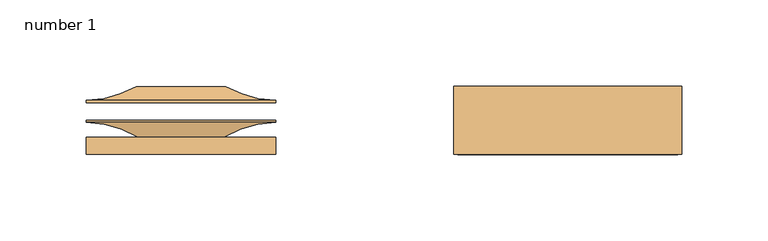
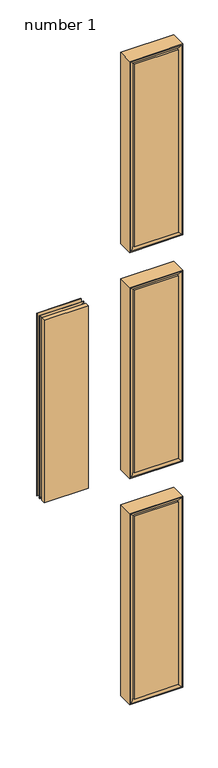
"""IFC4 building model written with IfcOpenShell, lengths in millimetres: door geometry, Door-Interior-Karona-K5660-6_Panel : number 1."""

from ifc_helpers import new_model, si_unit, frame, origin, place, context, project, spatial, polyline, ellipse_curve, source, transform, mapped, element, save
from ifc_brep_helpers import plane_surface, cylinder_surface, revolved_surface, advanced_brep


def number_1_6f4e57e8(model_context):
    return source(origin(), model_context, "Body", "AdvancedBrep", [
        advanced_brep(
        [(166.6748, -54.4576, 1893.8748), (57.1627, -54.4576, 1893.8748), (57.1627, -54.4576, 1414.4752), (166.6748, -54.4576, 1414.4752), (166.6748, -34.7218, 1893.8748), (57.1627, -34.7218, 1893.8748), (57.1627, -36.0454899, 1893.8748), (166.6748, -36.0454899, 1893.8748), (166.6748, -44.5515929, 1893.8748), (57.1627, -44.5515929, 1893.8748), (57.1627, -34.7218, 1414.4752), (166.6748, -34.7218, 1414.4752), (166.6748, -36.0454899, 1414.4752), (57.1627, -36.0454899, 1414.4752), (57.1627, -44.5515929, 1414.4752), (166.6748, -44.5515929, 1414.4752), (87.1686653, -44.5515929, 1863.8688347), (136.6688347, -44.5515929, 1863.8688347), (87.1686653, -44.5515929, 1444.4811653), (136.6688347, -44.5515929, 1444.4811653)],
        [
            (0, 1),
            (1, 2),
            (2, 3),
            (3, 0),
            (4, 5),
            (5, 6),
            (6, 7),
            (7, 4),
            (0, 8),
            (8, 9),
            (9, 1),
            (10, 11),
            (11, 12),
            (12, 13),
            (13, 10),
            (2, 14),
            (14, 15),
            (15, 3),
            (15, 8),
            (11, 4),
            (7, 12),
            (9, 14),
            (5, 10),
            (13, 6),
            (16, 17),
            (17, 7, ellipse_curve(frame((168.6131685, -100.0605261, 1895.8131685), z_axis=(0.7071067811865475, 0.0, -0.7071067811865475), x_axis=(0.7071067811865476, 0.0, 0.7071067811865474)), 90.5724254, 64.0443762)),
            (6, 16, ellipse_curve(frame((55.2243315, -100.0605261, 1895.8131685), z_axis=(-0.7071067811865475, 0.0, -0.7071067811865475), x_axis=(0.7071067811865476, 0.0, -0.7071067811865474)), 90.5724254, 64.0443762)),
            (18, 16),
            (13, 18, ellipse_curve(frame((55.2243315, -100.0605261, 1412.5368315), z_axis=(0.7071067811865475, 0.0, -0.7071067811865475), x_axis=(0.7071067811865474, 0.0, 0.7071067811865476)), 90.5724254, 64.0443762)),
            (19, 18),
            (12, 19, ellipse_curve(frame((168.6131685, -100.0605261, 1412.5368315), z_axis=(0.7071067811865475, 0.0, 0.7071067811865475), x_axis=(-0.7071067811865476, 0.0, 0.7071067811865474)), 90.5724254, 64.0443762)),
            (17, 19),
        ],
        [
            plane_surface(frame((57.1627, -54.4576, 1893.8748), z_axis=(0.0, -1.0, 0.0), x_axis=(0.0, 0.0, -1.0))),
            plane_surface(frame((57.1627, -34.7218, 1893.8748), z_axis=(0.0, 0.0, 1.0), x_axis=(-1.0, 0.0, 0.0))),
            plane_surface(frame((57.1627, -34.7218, 1414.4752), z_axis=(0.0, 0.0, -1.0), x_axis=(1.0, 0.0, 0.0))),
            plane_surface(frame((166.6748, -54.4576, 1893.8748), z_axis=(1.0, 0.0, 0.0), x_axis=(0.0, 0.0, -1.0))),
            plane_surface(frame((57.1627, -34.7218, 1893.8748), z_axis=(-1.0, 0.0, 0.0), x_axis=(0.0, 0.0, -1.0))),
            plane_surface(frame((166.6748, -34.7218, 1893.8748), z_axis=(0.0, 1.0, 0.0), x_axis=(0.0, 0.0, -1.0))),
            revolved_surface(polyline([(232.6575446888527, -100.0605261, 1831.7687923), (-8.820044688852704, -100.0605261, 1831.7687923)]), (177.8, -100.0605261, 1895.8131685), (1.0, 0.0, 0.0)),
            revolved_surface(polyline([(119.2687077, -100.0605261, 1959.8575446888528), (119.2687077, -100.0605261, 1348.4924553111473)]), (55.2243315, -100.0605261, 1905.0), (0.0, 0.0, 1.0)),
            revolved_surface(polyline([(-8.820044688852683, -100.0605261, 1476.5812077), (232.6575446888527, -100.0605261, 1476.5812077)]), (46.0375, -100.0605261, 1412.5368315), (-1.0, 0.0, 0.0)),
            revolved_surface(polyline([(104.5687923, -100.0605261, 1348.4924553111473), (104.5687923, -100.0605261, 1959.8575446888526)]), (168.6131685, -100.0605261, 1403.35), (0.0, 0.0, -1.0)),
            plane_surface(frame((177.8, -44.5515929, 1403.35), z_axis=(0.0, 1.0, 0.0), x_axis=(0.0, 0.0, 1.0))),
        ],
        [
            (0, [[1, 2, 3, 4]]),
            (1, [[5, 6, 7, 8]]),
            (1, [[-1, 9, 10, 11]]),
            (2, [[12, 13, 14, 15]]),
            (2, [[-3, 16, 17, 18]]),
            (3, [[-4, -18, 19, -9]]),
            (3, [[20, -8, 21, -13]]),
            (4, [[-2, -11, 22, -16]]),
            (4, [[23, -15, 24, -6]]),
            (5, [[-5, -20, -12, -23]]),
            (6, [[25, 26, -7, 27]]),
            (7, [[28, -27, -24, 29]]),
            (8, [[30, -29, -14, 31]]),
            (9, [[32, -31, -21, -26]]),
            (10, [[-10, -19, -17, -22], [-25, -28, -30, -32]]),
        ],
    ),
        advanced_brep(
        [(166.6748, -24.6126, 1893.8748), (57.1627, -24.6126, 1893.8748), (57.1627, -24.6126, 1414.4752), (166.6748, -24.6126, 1414.4752), (137.8448579, -15.4432, 1443.3051421), (85.9926421, -15.4432, 1443.3051421), (85.9926421, -15.4432, 1865.0448579), (137.8448579, -15.4432, 1865.0448579), (166.6748, -23.2889101, 1893.8748), (57.1627, -23.2889101, 1893.8748), (57.1627, -23.2889101, 1414.4752), (166.6748, -23.2889101, 1414.4752)],
        [
            (0, 1),
            (1, 2),
            (2, 3),
            (3, 0),
            (4, 5),
            (5, 6),
            (6, 7),
            (7, 4),
            (0, 8),
            (8, 9),
            (9, 1),
            (2, 10),
            (10, 11),
            (11, 3),
            (4, 11, ellipse_curve(frame((168.6131685, 40.7261261, 1412.5368315), z_axis=(0.7071067811865475, 0.0, 0.7071067811865475), x_axis=(-0.7071067811865476, 0.0, 0.7071067811865474)), 90.5724254, 64.0443762)),
            (10, 5, ellipse_curve(frame((55.2243315, 40.7261261, 1412.5368315), z_axis=(-0.7071067811865475, 0.0, 0.7071067811865475), x_axis=(-0.7071067811865476, 0.0, -0.7071067811865474)), 90.5724254, 64.0443762)),
            (7, 8, ellipse_curve(frame((168.6131685, 40.7261261, 1895.8131685), z_axis=(-0.7071067811865475, 0.0, 0.7071067811865475), x_axis=(-0.7071067811865474, 0.0, -0.7071067811865476)), 90.5724254, 64.0443762)),
            (8, 11),
            (6, 9, ellipse_curve(frame((55.2243315, 40.7261261, 1895.8131685), z_axis=(-0.7071067811865475, 0.0, -0.7071067811865475), x_axis=(0.7071067811865476, 0.0, -0.7071067811865474)), 90.5724254, 64.0443762)),
            (10, 9),
        ],
        [
            plane_surface(frame((57.1627, -24.6126, 1893.8748), z_axis=(0.0, -1.0, 0.0), x_axis=(0.0, 0.0, -1.0))),
            plane_surface(frame((166.6748, -15.4432, 1893.8748), z_axis=(0.0, 1.0, 0.0), x_axis=(0.0, 0.0, -1.0))),
            plane_surface(frame((57.1627, -34.7218, 1893.8748), z_axis=(0.0, 0.0, 1.0), x_axis=(-1.0, 0.0, 0.0))),
            plane_surface(frame((57.1627, -34.7218, 1414.4752), z_axis=(0.0, 0.0, -1.0), x_axis=(1.0, 0.0, 0.0))),
            revolved_surface(polyline([(-8.820044688852711, 40.7261261, 1476.5812077), (232.6575446888527, 40.7261261, 1476.5812077)]), (46.0375, 40.7261261, 1412.5368315), (-1.0, 0.0, 0.0)),
            revolved_surface(polyline([(104.5687923, 40.7261261, 1348.4924553111473), (104.5687923, 40.7261261, 1959.8575446888528)]), (168.6131685, 40.7261261, 1403.35), (0.0, 0.0, -1.0)),
            revolved_surface(polyline([(232.65754468885268, 40.7261261, 1831.7687923), (-8.820044688852704, 40.7261261, 1831.7687923)]), (177.8, 40.7261261, 1895.8131685), (1.0, 0.0, 0.0)),
            revolved_surface(polyline([(119.2687077, 40.7261261, 1959.8575446888528), (119.2687077, 40.7261261, 1348.4924553111473)]), (55.2243315, 40.7261261, 1905.0), (0.0, 0.0, 1.0)),
            plane_surface(frame((166.6748, -24.6126, 1893.8748), z_axis=(1.0, 0.0, 0.0), x_axis=(0.0, 0.0, -1.0))),
            plane_surface(frame((57.1627, -15.4432, 1893.8748), z_axis=(-1.0, 0.0, 0.0), x_axis=(0.0, 0.0, -1.0))),
        ],
        [
            (0, [[1, 2, 3, 4]]),
            (1, [[5, 6, 7, 8]]),
            (2, [[-1, 9, 10, 11]]),
            (3, [[-3, 12, 13, 14]]),
            (4, [[15, -13, 16, -5]]),
            (5, [[-15, -8, 17, 18]]),
            (6, [[-17, -7, 19, -10]]),
            (7, [[-19, -6, -16, 20]]),
            (8, [[-4, -14, -18, -9]]),
            (9, [[-2, -11, -20, -12]]),
        ],
    ),
        advanced_brep(
        [(177.8, -15.2908, 1905.0), (166.4746863, -24.6126, 1893.6746863), (57.3628137, -24.6126, 1893.6746863), (46.0375, -15.2908, 1905.0), (57.1627, -46.3324899, 1893.8748), (48.2727, -54.4576, 1902.7648), (48.2727, -54.4576, 1405.5852), (57.1627, -46.3324899, 1414.4752), (166.6748, -46.3324899, 1414.4752), (175.5648, -54.4576, 1405.5852), (175.5648, -54.4576, 1902.7648), (166.6748, -46.3324899, 1893.8748), (46.0375, -54.4576, 1403.35), (46.0375, -15.2908, 1403.35), (177.8, -15.2908, 1403.35), (177.8, -54.4576, 1403.35), (57.1627, -34.7218, 1414.4752), (166.6748, -34.7218, 1414.4752), (47.3075, -24.6126, 1903.73), (47.3075, -34.7218, 1903.73), (47.3075, -34.7218, 1404.62), (47.3075, -24.6126, 1404.62), (176.53, -24.6126, 1404.62), (176.53, -24.6126, 1903.73), (57.3628137, -24.6126, 1414.6753137), (166.4746863, -24.6126, 1414.6753137), (176.53, -34.7218, 1404.62), (177.8, -54.4576, 1905.0), (166.6748, -34.7218, 1893.8748), (176.53, -34.7218, 1903.73), (46.0375, -54.4576, 1905.0), (57.1627, -34.7218, 1893.8748)],
        [
            (0, 1, ellipse_curve(frame((176.7689876, -25.5788135, 1903.9689876), z_axis=(-0.7071067811865475, 0.0, 0.7071067811865475), x_axis=(0.7071067811865476, 0.0, 0.7071067811865474)), 14.6223259, 10.3395458)),
            (1, 2),
            (2, 3, ellipse_curve(frame((47.0685124, -25.5788135, 1903.9689876), z_axis=(0.7071067811865475, 0.0, 0.7071067811865475), x_axis=(0.7071067811865476, 0.0, -0.7071067811865474)), 14.6223259, 10.3395458)),
            (3, 0),
            (4, 5, ellipse_curve(frame((48.2727, -45.531597, 1902.7648), z_axis=(-0.7071067811865475, 0.0, -0.7071067811865475), x_axis=(-0.7071067811865474, 0.0, 0.7071067811865476)), 12.6232745, 8.926003)),
            (5, 6),
            (6, 7, ellipse_curve(frame((48.2727, -45.531597, 1405.5852), z_axis=(-0.7071067811865475, 0.0, 0.7071067811865475), x_axis=(0.7071067811865474, 0.0, 0.7071067811865476)), 12.6232745, 8.926003)),
            (7, 4),
            (8, 9, ellipse_curve(frame((175.5648, -45.531597, 1405.5852), z_axis=(0.7071067811865475, 0.0, 0.7071067811865475), x_axis=(0.7071067811865474, 0.0, -0.7071067811865476)), 12.6232745, 8.926003)),
            (9, 10),
            (10, 11, ellipse_curve(frame((175.5648, -45.531597, 1902.7648), z_axis=(0.7071067811865475, 0.0, -0.7071067811865475), x_axis=(-0.7071067811865474, 0.0, -0.7071067811865476)), 12.6232745, 8.926003)),
            (11, 8),
            (12, 13),
            (13, 14),
            (14, 15),
            (15, 12),
            (16, 7),
            (7, 8),
            (8, 17),
            (17, 16),
            (18, 19),
            (19, 20),
            (20, 21),
            (21, 18),
            (22, 23),
            (23, 18),
            (21, 22),
            (24, 2),
            (1, 25),
            (25, 24),
            (20, 26),
            (26, 22),
            (14, 0),
            (0, 27),
            (27, 15),
            (11, 28),
            (28, 17),
            (26, 29),
            (29, 23),
            (3, 30),
            (30, 27),
            (11, 4),
            (4, 31),
            (31, 28),
            (29, 19),
            (3, 13),
            (12, 30),
            (16, 31),
            (5, 10),
            (9, 6),
            (13, 24, ellipse_curve(frame((47.0685124, -25.5788135, 1404.3810124), z_axis=(0.7071067811865475, 0.0, -0.7071067811865475), x_axis=(-0.7071067811865476, 0.0, -0.7071067811865474)), 14.6223259, 10.3395458)),
            (25, 14, ellipse_curve(frame((176.7689876, -25.5788135, 1404.3810124), z_axis=(-0.7071067811865475, 0.0, -0.7071067811865475), x_axis=(-0.7071067811865476, 0.0, 0.7071067811865474)), 14.6223259, 10.3395458)),
        ],
        [
            cylinder_surface(frame((177.8, -25.5788135, 1903.9689876), z_axis=(1.0, 0.0, 0.0), x_axis=(0.0, 1.0, 0.0)), 10.3395458),
            cylinder_surface(frame((48.2727, -45.531597, 1905.0), z_axis=(0.0, 0.0, 1.0), x_axis=(0.0, 1.0, 0.0)), 8.926003),
            cylinder_surface(frame((175.5648, -45.531597, 1403.35), z_axis=(0.0, 0.0, -1.0), x_axis=(0.0, 1.0, 0.0)), 8.926003),
            plane_surface(frame((46.0375, -15.2908, 1403.35), z_axis=(0.0, 0.0, -1.0), x_axis=(1.0, 0.0, 0.0))),
            plane_surface(frame((57.1627, -46.3324899, 1414.4752), z_axis=(0.0, 0.0, 1.0), x_axis=(1.0, 0.0, 0.0))),
            plane_surface(frame((47.3075, -34.7218, 1903.73), z_axis=(1.0, 0.0, 0.0), x_axis=(0.0, 0.0, -1.0))),
            plane_surface(frame((47.3075, -24.6126, 1903.73), z_axis=(0.0, -1.0, 0.0), x_axis=(0.0, 0.0, -1.0))),
            plane_surface(frame((47.3075, -34.7218, 1404.62), z_axis=(0.0, 0.0, 1.0), x_axis=(1.0, 0.0, 0.0))),
            plane_surface(frame((177.8, -15.2908, 1403.35), z_axis=(1.0, 0.0, 0.0), x_axis=(0.0, 0.0, 1.0))),
            plane_surface(frame((166.6748, -46.3324899, 1414.4752), z_axis=(-1.0, 0.0, 0.0), x_axis=(0.0, 0.0, 1.0))),
            plane_surface(frame((176.53, -34.7218, 1404.62), z_axis=(-1.0, 0.0, 0.0), x_axis=(0.0, 0.0, 1.0))),
            plane_surface(frame((177.8, -15.2908, 1905.0), z_axis=(0.0, 0.0, 1.0), x_axis=(-1.0, 0.0, 0.0))),
            plane_surface(frame((166.6748, -46.3324899, 1893.8748), z_axis=(0.0, 0.0, -1.0), x_axis=(-1.0, 0.0, 0.0))),
            plane_surface(frame((176.53, -34.7218, 1903.73), z_axis=(0.0, 0.0, -1.0), x_axis=(-1.0, 0.0, 0.0))),
            plane_surface(frame((46.0375, -15.2908, 1905.0), z_axis=(-1.0, 0.0, 0.0), x_axis=(0.0, 0.0, -1.0))),
            plane_surface(frame((57.1627, -46.3324899, 1893.8748), z_axis=(1.0, 0.0, 0.0), x_axis=(0.0, 0.0, -1.0))),
            plane_surface(frame((57.1627, -34.7218, 1893.8748), z_axis=(0.0, 1.0, 0.0), x_axis=(0.0, 0.0, -1.0))),
            plane_surface(frame((46.0375, -54.4576, 1905.0), z_axis=(0.0, -1.0, 0.0), x_axis=(0.0, 0.0, -1.0))),
            cylinder_surface(frame((46.0375, -45.531597, 1405.5852), z_axis=(-1.0, 0.0, 0.0), x_axis=(0.0, 1.0, 0.0)), 8.926003),
            cylinder_surface(frame((46.0375, -25.5788135, 1404.3810124), z_axis=(-1.0, 0.0, 0.0), x_axis=(0.0, 1.0, 0.0)), 10.3395458),
            cylinder_surface(frame((176.7689876, -25.5788135, 1403.35), z_axis=(0.0, 0.0, -1.0), x_axis=(0.0, 1.0, 0.0)), 10.3395458),
            cylinder_surface(frame((177.8, -45.531597, 1902.7648), z_axis=(1.0, 0.0, 0.0), x_axis=(0.0, 1.0, 0.0)), 8.926003),
            cylinder_surface(frame((47.0685124, -25.5788135, 1905.0), z_axis=(0.0, 0.0, 1.0), x_axis=(0.0, 1.0, 0.0)), 10.3395458),
        ],
        [
            (0, [[1, 2, 3, 4]]),
            (1, [[5, 6, 7, 8]]),
            (2, [[9, 10, 11, 12]]),
            (3, [[13, 14, 15, 16]]),
            (4, [[17, 18, 19, 20]]),
            (5, [[21, 22, 23, 24]]),
            (6, [[25, 26, -24, 27], [28, -2, 29, 30]]),
            (7, [[-23, 31, 32, -27]]),
            (8, [[-15, 33, 34, 35]]),
            (9, [[-19, -12, 36, 37]]),
            (10, [[-32, 38, 39, -25]]),
            (11, [[-34, -4, 40, 41]]),
            (12, [[-36, 42, 43, 44]]),
            (13, [[-39, 45, -21, -26]]),
            (14, [[-40, 46, -13, 47]]),
            (15, [[-43, -8, -17, 48]]),
            (16, [[-22, -45, -38, -31], [-37, -44, -48, -20]]),
            (17, [[-35, -41, -47, -16], [-6, 49, -10, 50]]),
            (18, [[-7, -50, -9, -18]]),
            (19, [[51, -30, 52, -14]]),
            (20, [[-52, -29, -1, -33]]),
            (21, [[-11, -49, -5, -42]]),
            (22, [[-3, -28, -51, -46]]),
        ],
    ),
        advanced_brep(
        [(166.6748, -54.4576, 1300.1498), (57.1627, -54.4576, 1300.1498), (57.1627, -54.4576, 820.7502), (166.6748, -54.4576, 820.7502), (166.6748, -34.7218, 1300.1498), (57.1627, -34.7218, 1300.1498), (57.1627, -36.0454899, 1300.1498), (166.6748, -36.0454899, 1300.1498), (166.6748, -44.5515929, 1300.1498), (57.1627, -44.5515929, 1300.1498), (57.1627, -34.7218, 820.7502), (166.6748, -34.7218, 820.7502), (166.6748, -36.0454899, 820.7502), (57.1627, -36.0454899, 820.7502), (57.1627, -44.5515929, 820.7502), (166.6748, -44.5515929, 820.7502), (87.1686653, -44.5515929, 1270.1438347), (136.6688347, -44.5515929, 1270.1438347), (87.1686653, -44.5515929, 850.7561653), (136.6688347, -44.5515929, 850.7561653)],
        [
            (0, 1),
            (1, 2),
            (2, 3),
            (3, 0),
            (4, 5),
            (5, 6),
            (6, 7),
            (7, 4),
            (0, 8),
            (8, 9),
            (9, 1),
            (10, 11),
            (11, 12),
            (12, 13),
            (13, 10),
            (2, 14),
            (14, 15),
            (15, 3),
            (15, 8),
            (11, 4),
            (7, 12),
            (9, 14),
            (5, 10),
            (13, 6),
            (16, 17),
            (17, 7, ellipse_curve(frame((168.6131685, -100.0605261, 1302.0881685), z_axis=(0.7071067811865475, 0.0, -0.7071067811865475), x_axis=(0.7071067811865476, 0.0, 0.7071067811865474)), 90.5724254, 64.0443762)),
            (6, 16, ellipse_curve(frame((55.2243315, -100.0605261, 1302.0881685), z_axis=(-0.7071067811865475, 0.0, -0.7071067811865475), x_axis=(0.7071067811865476, 0.0, -0.7071067811865474)), 90.5724254, 64.0443762)),
            (18, 16),
            (13, 18, ellipse_curve(frame((55.2243315, -100.0605261, 818.8118315), z_axis=(0.7071067811865475, 0.0, -0.7071067811865475), x_axis=(0.7071067811865474, 0.0, 0.7071067811865476)), 90.5724254, 64.0443762)),
            (19, 18),
            (12, 19, ellipse_curve(frame((168.6131685, -100.0605261, 818.8118315), z_axis=(0.7071067811865475, 0.0, 0.7071067811865475), x_axis=(-0.7071067811865476, 0.0, 0.7071067811865474)), 90.5724254, 64.0443762)),
            (17, 19),
        ],
        [
            plane_surface(frame((57.1627, -54.4576, 1300.1498), z_axis=(0.0, -1.0, 0.0), x_axis=(0.0, 0.0, -1.0))),
            plane_surface(frame((57.1627, -34.7218, 1300.1498), z_axis=(0.0, 0.0, 1.0), x_axis=(-1.0, 0.0, 0.0))),
            plane_surface(frame((57.1627, -34.7218, 820.7502), z_axis=(0.0, 0.0, -1.0), x_axis=(1.0, 0.0, 0.0))),
            plane_surface(frame((166.6748, -54.4576, 1300.1498), z_axis=(1.0, 0.0, 0.0), x_axis=(0.0, 0.0, -1.0))),
            plane_surface(frame((57.1627, -34.7218, 1300.1498), z_axis=(-1.0, 0.0, 0.0), x_axis=(0.0, 0.0, -1.0))),
            plane_surface(frame((166.6748, -34.7218, 1300.1498), z_axis=(0.0, 1.0, 0.0), x_axis=(0.0, 0.0, -1.0))),
            revolved_surface(polyline([(232.6575446888527, -100.0605261, 1238.0437923), (-8.820044688852704, -100.0605261, 1238.0437923)]), (177.8, -100.0605261, 1302.0881685), (1.0, 0.0, 0.0)),
            revolved_surface(polyline([(119.2687077, -100.0605261, 1366.1325446888527), (119.2687077, -100.0605261, 754.7674553111474)]), (55.2243315, -100.0605261, 1311.275), (0.0, 0.0, 1.0)),
            revolved_surface(polyline([(-8.820044688852683, -100.0605261, 882.8562077), (232.6575446888527, -100.0605261, 882.8562077)]), (46.0375, -100.0605261, 818.8118315), (-1.0, 0.0, 0.0)),
            revolved_surface(polyline([(104.5687923, -100.0605261, 754.7674553111474), (104.5687923, -100.0605261, 1366.1325446888527)]), (168.6131685, -100.0605261, 809.625), (0.0, 0.0, -1.0)),
            plane_surface(frame((177.8, -44.5515929, 809.625), z_axis=(0.0, 1.0, 0.0), x_axis=(0.0, 0.0, 1.0))),
        ],
        [
            (0, [[1, 2, 3, 4]]),
            (1, [[5, 6, 7, 8]]),
            (1, [[-1, 9, 10, 11]]),
            (2, [[12, 13, 14, 15]]),
            (2, [[-3, 16, 17, 18]]),
            (3, [[-4, -18, 19, -9]]),
            (3, [[20, -8, 21, -13]]),
            (4, [[-2, -11, 22, -16]]),
            (4, [[23, -15, 24, -6]]),
            (5, [[-5, -20, -12, -23]]),
            (6, [[25, 26, -7, 27]]),
            (7, [[28, -27, -24, 29]]),
            (8, [[30, -29, -14, 31]]),
            (9, [[32, -31, -21, -26]]),
            (10, [[-10, -19, -17, -22], [-25, -28, -30, -32]]),
        ],
    ),
        advanced_brep(
        [(166.6748, -24.6126, 1300.1498), (57.1627, -24.6126, 1300.1498), (57.1627, -24.6126, 820.7502), (166.6748, -24.6126, 820.7502), (137.8448579, -15.4432, 849.5801421), (85.9926421, -15.4432, 849.5801421), (85.9926421, -15.4432, 1271.3198579), (137.8448579, -15.4432, 1271.3198579), (166.6748, -23.2889101, 1300.1498), (57.1627, -23.2889101, 1300.1498), (57.1627, -23.2889101, 820.7502), (166.6748, -23.2889101, 820.7502)],
        [
            (0, 1),
            (1, 2),
            (2, 3),
            (3, 0),
            (4, 5),
            (5, 6),
            (6, 7),
            (7, 4),
            (0, 8),
            (8, 9),
            (9, 1),
            (2, 10),
            (10, 11),
            (11, 3),
            (4, 11, ellipse_curve(frame((168.6131685, 40.7261261, 818.8118315), z_axis=(0.7071067811865475, 0.0, 0.7071067811865475), x_axis=(-0.7071067811865476, 0.0, 0.7071067811865474)), 90.5724254, 64.0443762)),
            (10, 5, ellipse_curve(frame((55.2243315, 40.7261261, 818.8118315), z_axis=(-0.7071067811865475, 0.0, 0.7071067811865475), x_axis=(-0.7071067811865476, 0.0, -0.7071067811865474)), 90.5724254, 64.0443762)),
            (7, 8, ellipse_curve(frame((168.6131685, 40.7261261, 1302.0881685), z_axis=(-0.7071067811865475, 0.0, 0.7071067811865475), x_axis=(-0.7071067811865474, 0.0, -0.7071067811865476)), 90.5724254, 64.0443762)),
            (8, 11),
            (6, 9, ellipse_curve(frame((55.2243315, 40.7261261, 1302.0881685), z_axis=(-0.7071067811865475, 0.0, -0.7071067811865475), x_axis=(0.7071067811865476, 0.0, -0.7071067811865474)), 90.5724254, 64.0443762)),
            (10, 9),
        ],
        [
            plane_surface(frame((57.1627, -24.6126, 1300.1498), z_axis=(0.0, -1.0, 0.0), x_axis=(0.0, 0.0, -1.0))),
            plane_surface(frame((166.6748, -15.4432, 1300.1498), z_axis=(0.0, 1.0, 0.0), x_axis=(0.0, 0.0, -1.0))),
            plane_surface(frame((57.1627, -34.7218, 1300.1498), z_axis=(0.0, 0.0, 1.0), x_axis=(-1.0, 0.0, 0.0))),
            plane_surface(frame((57.1627, -34.7218, 820.7502), z_axis=(0.0, 0.0, -1.0), x_axis=(1.0, 0.0, 0.0))),
            revolved_surface(polyline([(-8.820044688852711, 40.7261261, 882.8562077), (232.6575446888527, 40.7261261, 882.8562077)]), (46.0375, 40.7261261, 818.8118315), (-1.0, 0.0, 0.0)),
            revolved_surface(polyline([(104.5687923, 40.7261261, 754.7674553111474), (104.5687923, 40.7261261, 1366.1325446888527)]), (168.6131685, 40.7261261, 809.625), (0.0, 0.0, -1.0)),
            revolved_surface(polyline([(232.65754468885268, 40.7261261, 1238.0437923), (-8.820044688852704, 40.7261261, 1238.0437923)]), (177.8, 40.7261261, 1302.0881685), (1.0, 0.0, 0.0)),
            revolved_surface(polyline([(119.2687077, 40.7261261, 1366.1325446888527), (119.2687077, 40.7261261, 754.7674553111474)]), (55.2243315, 40.7261261, 1311.275), (0.0, 0.0, 1.0)),
            plane_surface(frame((166.6748, -24.6126, 1300.1498), z_axis=(1.0, 0.0, 0.0), x_axis=(0.0, 0.0, -1.0))),
            plane_surface(frame((57.1627, -15.4432, 1300.1498), z_axis=(-1.0, 0.0, 0.0), x_axis=(0.0, 0.0, -1.0))),
        ],
        [
            (0, [[1, 2, 3, 4]]),
            (1, [[5, 6, 7, 8]]),
            (2, [[-1, 9, 10, 11]]),
            (3, [[-3, 12, 13, 14]]),
            (4, [[15, -13, 16, -5]]),
            (5, [[-15, -8, 17, 18]]),
            (6, [[-17, -7, 19, -10]]),
            (7, [[-19, -6, -16, 20]]),
            (8, [[-4, -14, -18, -9]]),
            (9, [[-2, -11, -20, -12]]),
        ],
    ),
        advanced_brep(
        [(177.8, -15.2908, 1311.275), (166.4746863, -24.6126, 1299.9496863), (57.3628137, -24.6126, 1299.9496863), (46.0375, -15.2908, 1311.275), (57.1627, -46.3324899, 1300.1498), (48.2727, -54.4576, 1309.0398), (48.2727, -54.4576, 811.8602), (57.1627, -46.3324899, 820.7502), (166.6748, -46.3324899, 820.7502), (175.5648, -54.4576, 811.8602), (175.5648, -54.4576, 1309.0398), (166.6748, -46.3324899, 1300.1498), (46.0375, -54.4576, 809.625), (46.0375, -15.2908, 809.625), (177.8, -15.2908, 809.625), (177.8, -54.4576, 809.625), (57.1627, -34.7218, 820.7502), (166.6748, -34.7218, 820.7502), (47.3075, -24.6126, 1310.005), (47.3075, -34.7218, 1310.005), (47.3075, -34.7218, 810.895), (47.3075, -24.6126, 810.895), (176.53, -24.6126, 810.895), (176.53, -24.6126, 1310.005), (57.3628137, -24.6126, 820.9503137), (166.4746863, -24.6126, 820.9503137), (176.53, -34.7218, 810.895), (177.8, -54.4576, 1311.275), (166.6748, -34.7218, 1300.1498), (176.53, -34.7218, 1310.005), (46.0375, -54.4576, 1311.275), (57.1627, -34.7218, 1300.1498)],
        [
            (0, 1, ellipse_curve(frame((176.7689876, -25.5788135, 1310.2439876), z_axis=(-0.7071067811865475, 0.0, 0.7071067811865475), x_axis=(0.7071067811865476, 0.0, 0.7071067811865474)), 14.6223259, 10.3395458)),
            (1, 2),
            (2, 3, ellipse_curve(frame((47.0685124, -25.5788135, 1310.2439876), z_axis=(0.7071067811865475, 0.0, 0.7071067811865475), x_axis=(0.7071067811865476, 0.0, -0.7071067811865474)), 14.6223259, 10.3395458)),
            (3, 0),
            (4, 5, ellipse_curve(frame((48.2727, -45.531597, 1309.0398), z_axis=(-0.7071067811865475, 0.0, -0.7071067811865475), x_axis=(-0.7071067811865474, 0.0, 0.7071067811865476)), 12.6232745, 8.926003)),
            (5, 6),
            (6, 7, ellipse_curve(frame((48.2727, -45.531597, 811.8602), z_axis=(-0.7071067811865475, 0.0, 0.7071067811865475), x_axis=(0.7071067811865474, 0.0, 0.7071067811865476)), 12.6232745, 8.926003)),
            (7, 4),
            (8, 9, ellipse_curve(frame((175.5648, -45.531597, 811.8602), z_axis=(0.7071067811865475, 0.0, 0.7071067811865475), x_axis=(0.7071067811865474, 0.0, -0.7071067811865476)), 12.6232745, 8.926003)),
            (9, 10),
            (10, 11, ellipse_curve(frame((175.5648, -45.531597, 1309.0398), z_axis=(0.7071067811865475, 0.0, -0.7071067811865475), x_axis=(-0.7071067811865474, 0.0, -0.7071067811865476)), 12.6232745, 8.926003)),
            (11, 8),
            (12, 13),
            (13, 14),
            (14, 15),
            (15, 12),
            (16, 7),
            (7, 8),
            (8, 17),
            (17, 16),
            (18, 19),
            (19, 20),
            (20, 21),
            (21, 18),
            (22, 23),
            (23, 18),
            (21, 22),
            (24, 2),
            (1, 25),
            (25, 24),
            (13, 24, ellipse_curve(frame((47.0685124, -25.5788135, 810.6560124), z_axis=(0.7071067811865475, 0.0, -0.7071067811865475), x_axis=(-0.7071067811865476, 0.0, -0.7071067811865474)), 14.6223259, 10.3395458)),
            (25, 14, ellipse_curve(frame((176.7689876, -25.5788135, 810.6560124), z_axis=(-0.7071067811865475, 0.0, -0.7071067811865475), x_axis=(-0.7071067811865476, 0.0, 0.7071067811865474)), 14.6223259, 10.3395458)),
            (20, 26),
            (26, 22),
            (14, 0),
            (0, 27),
            (27, 15),
            (11, 28),
            (28, 17),
            (26, 29),
            (29, 23),
            (3, 30),
            (30, 27),
            (11, 4),
            (4, 31),
            (31, 28),
            (29, 19),
            (3, 13),
            (12, 30),
            (16, 31),
            (5, 10),
            (9, 6),
        ],
        [
            cylinder_surface(frame((177.8, -25.5788135, 1310.2439876), z_axis=(1.0, 0.0, 0.0), x_axis=(0.0, 1.0, 0.0)), 10.3395458),
            cylinder_surface(frame((48.2727, -45.531597, 1311.275), z_axis=(0.0, 0.0, 1.0), x_axis=(0.0, 1.0, 0.0)), 8.926003),
            cylinder_surface(frame((175.5648, -45.531597, 809.625), z_axis=(0.0, 0.0, -1.0), x_axis=(0.0, 1.0, 0.0)), 8.926003),
            plane_surface(frame((46.0375, -15.2908, 809.625), z_axis=(0.0, 0.0, -1.0), x_axis=(1.0, 0.0, 0.0))),
            plane_surface(frame((57.1627, -46.3324899, 820.7502), z_axis=(0.0, 0.0, 1.0), x_axis=(1.0, 0.0, 0.0))),
            plane_surface(frame((47.3075, -34.7218, 1310.005), z_axis=(1.0, 0.0, 0.0), x_axis=(0.0, 0.0, -1.0))),
            plane_surface(frame((47.3075, -24.6126, 1310.005), z_axis=(0.0, -1.0, 0.0), x_axis=(0.0, 0.0, -1.0))),
            cylinder_surface(frame((46.0375, -25.5788135, 810.6560124), z_axis=(-1.0, 0.0, 0.0), x_axis=(0.0, 1.0, 0.0)), 10.3395458),
            plane_surface(frame((47.3075, -34.7218, 810.895), z_axis=(0.0, 0.0, 1.0), x_axis=(1.0, 0.0, 0.0))),
            plane_surface(frame((177.8, -15.2908, 809.625), z_axis=(1.0, 0.0, 0.0), x_axis=(0.0, 0.0, 1.0))),
            plane_surface(frame((166.6748, -46.3324899, 820.7502), z_axis=(-1.0, 0.0, 0.0), x_axis=(0.0, 0.0, 1.0))),
            plane_surface(frame((176.53, -34.7218, 810.895), z_axis=(-1.0, 0.0, 0.0), x_axis=(0.0, 0.0, 1.0))),
            plane_surface(frame((177.8, -15.2908, 1311.275), z_axis=(0.0, 0.0, 1.0), x_axis=(-1.0, 0.0, 0.0))),
            plane_surface(frame((166.6748, -46.3324899, 1300.1498), z_axis=(0.0, 0.0, -1.0), x_axis=(-1.0, 0.0, 0.0))),
            plane_surface(frame((176.53, -34.7218, 1310.005), z_axis=(0.0, 0.0, -1.0), x_axis=(-1.0, 0.0, 0.0))),
            plane_surface(frame((46.0375, -15.2908, 1311.275), z_axis=(-1.0, 0.0, 0.0), x_axis=(0.0, 0.0, -1.0))),
            plane_surface(frame((57.1627, -46.3324899, 1300.1498), z_axis=(1.0, 0.0, 0.0), x_axis=(0.0, 0.0, -1.0))),
            plane_surface(frame((57.1627, -34.7218, 1300.1498), z_axis=(0.0, 1.0, 0.0), x_axis=(0.0, 0.0, -1.0))),
            plane_surface(frame((46.0375, -54.4576, 1311.275), z_axis=(0.0, -1.0, 0.0), x_axis=(0.0, 0.0, -1.0))),
            cylinder_surface(frame((46.0375, -45.531597, 811.8602), z_axis=(-1.0, 0.0, 0.0), x_axis=(0.0, 1.0, 0.0)), 8.926003),
            cylinder_surface(frame((176.7689876, -25.5788135, 809.625), z_axis=(0.0, 0.0, -1.0), x_axis=(0.0, 1.0, 0.0)), 10.3395458),
            cylinder_surface(frame((177.8, -45.531597, 1309.0398), z_axis=(1.0, 0.0, 0.0), x_axis=(0.0, 1.0, 0.0)), 8.926003),
            cylinder_surface(frame((47.0685124, -25.5788135, 1311.275), z_axis=(0.0, 0.0, 1.0), x_axis=(0.0, 1.0, 0.0)), 10.3395458),
        ],
        [
            (0, [[1, 2, 3, 4]]),
            (1, [[5, 6, 7, 8]]),
            (2, [[9, 10, 11, 12]]),
            (3, [[13, 14, 15, 16]]),
            (4, [[17, 18, 19, 20]]),
            (5, [[21, 22, 23, 24]]),
            (6, [[25, 26, -24, 27], [28, -2, 29, 30]]),
            (7, [[31, -30, 32, -14]]),
            (8, [[-23, 33, 34, -27]]),
            (9, [[-15, 35, 36, 37]]),
            (10, [[-19, -12, 38, 39]]),
            (11, [[-34, 40, 41, -25]]),
            (12, [[-36, -4, 42, 43]]),
            (13, [[-38, 44, 45, 46]]),
            (14, [[-41, 47, -21, -26]]),
            (15, [[-42, 48, -13, 49]]),
            (16, [[-45, -8, -17, 50]]),
            (17, [[-22, -47, -40, -33], [-39, -46, -50, -20]]),
            (18, [[-37, -43, -49, -16], [-6, 51, -10, 52]]),
            (19, [[-7, -52, -9, -18]]),
            (20, [[-32, -29, -1, -35]]),
            (21, [[-11, -51, -5, -44]]),
            (22, [[-3, -28, -31, -48]]),
        ],
    ),
        advanced_brep(
        [(166.6748, -54.4576, 706.4248), (57.1627, -54.4576, 706.4248), (57.1627, -54.4576, 227.0252), (166.6748, -54.4576, 227.0252), (166.6748, -34.7218, 706.4248), (57.1627, -34.7218, 706.4248), (57.1627, -36.0454899, 706.4248), (166.6748, -36.0454899, 706.4248), (166.6748, -44.5515929, 706.4248), (57.1627, -44.5515929, 706.4248), (57.1627, -34.7218, 227.0252), (166.6748, -34.7218, 227.0252), (166.6748, -36.0454899, 227.0252), (57.1627, -36.0454899, 227.0252), (57.1627, -44.5515929, 227.0252), (166.6748, -44.5515929, 227.0252), (87.1686653, -44.5515929, 676.4188347), (136.6688347, -44.5515929, 676.4188347), (87.1686653, -44.5515929, 257.0311653), (136.6688347, -44.5515929, 257.0311653)],
        [
            (0, 1),
            (1, 2),
            (2, 3),
            (3, 0),
            (4, 5),
            (5, 6),
            (6, 7),
            (7, 4),
            (0, 8),
            (8, 9),
            (9, 1),
            (10, 11),
            (11, 12),
            (12, 13),
            (13, 10),
            (2, 14),
            (14, 15),
            (15, 3),
            (15, 8),
            (11, 4),
            (7, 12),
            (9, 14),
            (5, 10),
            (13, 6),
            (16, 17),
            (17, 7, ellipse_curve(frame((168.6131685, -100.0605261, 708.3631685), z_axis=(0.7071067811865475, 0.0, -0.7071067811865475), x_axis=(0.7071067811865476, 0.0, 0.7071067811865474)), 90.5724254, 64.0443762)),
            (6, 16, ellipse_curve(frame((55.2243315, -100.0605261, 708.3631685), z_axis=(-0.7071067811865475, 0.0, -0.7071067811865475), x_axis=(0.7071067811865476, 0.0, -0.7071067811865474)), 90.5724254, 64.0443762)),
            (18, 16),
            (13, 18, ellipse_curve(frame((55.2243315, -100.0605261, 225.0868315), z_axis=(0.7071067811865475, 0.0, -0.7071067811865475), x_axis=(0.7071067811865474, 0.0, 0.7071067811865476)), 90.5724254, 64.0443762)),
            (19, 18),
            (12, 19, ellipse_curve(frame((168.6131685, -100.0605261, 225.0868315), z_axis=(0.7071067811865475, 0.0, 0.7071067811865475), x_axis=(-0.7071067811865476, 0.0, 0.7071067811865474)), 90.5724254, 64.0443762)),
            (17, 19),
        ],
        [
            plane_surface(frame((57.1627, -54.4576, 706.4248), z_axis=(0.0, -1.0, 0.0), x_axis=(0.0, 0.0, -1.0))),
            plane_surface(frame((57.1627, -34.7218, 706.4248), z_axis=(0.0, 0.0, 1.0), x_axis=(-1.0, 0.0, 0.0))),
            plane_surface(frame((57.1627, -34.7218, 227.0252), z_axis=(0.0, 0.0, -1.0), x_axis=(1.0, 0.0, 0.0))),
            plane_surface(frame((166.6748, -54.4576, 706.4248), z_axis=(1.0, 0.0, 0.0), x_axis=(0.0, 0.0, -1.0))),
            plane_surface(frame((57.1627, -34.7218, 706.4248), z_axis=(-1.0, 0.0, 0.0), x_axis=(0.0, 0.0, -1.0))),
            plane_surface(frame((166.6748, -34.7218, 706.4248), z_axis=(0.0, 1.0, 0.0), x_axis=(0.0, 0.0, -1.0))),
            revolved_surface(polyline([(232.6575446888527, -100.0605261, 644.3187923), (-8.820044688852704, -100.0605261, 644.3187923)]), (177.8, -100.0605261, 708.3631685), (1.0, 0.0, 0.0)),
            revolved_surface(polyline([(119.2687077, -100.0605261, 772.4075446888527), (119.2687077, -100.0605261, 161.04245531114725)]), (55.2243315, -100.0605261, 717.55), (0.0, 0.0, 1.0)),
            revolved_surface(polyline([(-8.820044688852683, -100.0605261, 289.1312077), (232.6575446888527, -100.0605261, 289.1312077)]), (46.0375, -100.0605261, 225.0868315), (-1.0, 0.0, 0.0)),
            revolved_surface(polyline([(104.5687923, -100.0605261, 161.0424553111473), (104.5687923, -100.0605261, 772.4075446888527)]), (168.6131685, -100.0605261, 215.9), (0.0, 0.0, -1.0)),
            plane_surface(frame((177.8, -44.5515929, 215.9), z_axis=(0.0, 1.0, 0.0), x_axis=(0.0, 0.0, 1.0))),
        ],
        [
            (0, [[1, 2, 3, 4]]),
            (1, [[5, 6, 7, 8]]),
            (1, [[-1, 9, 10, 11]]),
            (2, [[12, 13, 14, 15]]),
            (2, [[-3, 16, 17, 18]]),
            (3, [[-4, -18, 19, -9]]),
            (3, [[20, -8, 21, -13]]),
            (4, [[-2, -11, 22, -16]]),
            (4, [[23, -15, 24, -6]]),
            (5, [[-5, -20, -12, -23]]),
            (6, [[25, 26, -7, 27]]),
            (7, [[28, -27, -24, 29]]),
            (8, [[30, -29, -14, 31]]),
            (9, [[32, -31, -21, -26]]),
            (10, [[-10, -19, -17, -22], [-25, -28, -30, -32]]),
        ],
    ),
        advanced_brep(
        [(166.6748, -24.6126, 706.4248), (57.1627, -24.6126, 706.4248), (57.1627, -24.6126, 227.0252), (166.6748, -24.6126, 227.0252), (137.8448579, -15.4432, 255.8551421), (85.9926421, -15.4432, 255.8551421), (85.9926421, -15.4432, 677.5948579), (137.8448579, -15.4432, 677.5948579), (166.6748, -23.2889101, 706.4248), (57.1627, -23.2889101, 706.4248), (57.1627, -23.2889101, 227.0252), (166.6748, -23.2889101, 227.0252)],
        [
            (0, 1),
            (1, 2),
            (2, 3),
            (3, 0),
            (4, 5),
            (5, 6),
            (6, 7),
            (7, 4),
            (0, 8),
            (8, 9),
            (9, 1),
            (2, 10),
            (10, 11),
            (11, 3),
            (4, 11, ellipse_curve(frame((168.6131685, 40.7261261, 225.0868315), z_axis=(0.7071067811865475, 0.0, 0.7071067811865475), x_axis=(-0.7071067811865476, 0.0, 0.7071067811865474)), 90.5724254, 64.0443762)),
            (10, 5, ellipse_curve(frame((55.2243315, 40.7261261, 225.0868315), z_axis=(-0.7071067811865475, 0.0, 0.7071067811865475), x_axis=(-0.7071067811865476, 0.0, -0.7071067811865474)), 90.5724254, 64.0443762)),
            (7, 8, ellipse_curve(frame((168.6131685, 40.7261261, 708.3631685), z_axis=(-0.7071067811865475, 0.0, 0.7071067811865475), x_axis=(-0.7071067811865474, 0.0, -0.7071067811865476)), 90.5724254, 64.0443762)),
            (8, 11),
            (6, 9, ellipse_curve(frame((55.2243315, 40.7261261, 708.3631685), z_axis=(-0.7071067811865475, 0.0, -0.7071067811865475), x_axis=(0.7071067811865476, 0.0, -0.7071067811865474)), 90.5724254, 64.0443762)),
            (10, 9),
        ],
        [
            plane_surface(frame((57.1627, -24.6126, 706.4248), z_axis=(0.0, -1.0, 0.0), x_axis=(0.0, 0.0, -1.0))),
            plane_surface(frame((166.6748, -15.4432, 706.4248), z_axis=(0.0, 1.0, 0.0), x_axis=(0.0, 0.0, -1.0))),
            plane_surface(frame((57.1627, -34.7218, 706.4248), z_axis=(0.0, 0.0, 1.0), x_axis=(-1.0, 0.0, 0.0))),
            plane_surface(frame((57.1627, -34.7218, 227.0252), z_axis=(0.0, 0.0, -1.0), x_axis=(1.0, 0.0, 0.0))),
            revolved_surface(polyline([(-8.820044688852711, 40.7261261, 289.1312077), (232.6575446888527, 40.7261261, 289.1312077)]), (46.0375, 40.7261261, 225.0868315), (-1.0, 0.0, 0.0)),
            revolved_surface(polyline([(104.5687923, 40.7261261, 161.0424553111473), (104.5687923, 40.7261261, 772.4075446888527)]), (168.6131685, 40.7261261, 215.9), (0.0, 0.0, -1.0)),
            revolved_surface(polyline([(232.65754468885268, 40.7261261, 644.3187923), (-8.820044688852704, 40.7261261, 644.3187923)]), (177.8, 40.7261261, 708.3631685), (1.0, 0.0, 0.0)),
            revolved_surface(polyline([(119.2687077, 40.7261261, 772.4075446888527), (119.2687077, 40.7261261, 161.04245531114736)]), (55.2243315, 40.7261261, 717.55), (0.0, 0.0, 1.0)),
            plane_surface(frame((166.6748, -24.6126, 706.4248), z_axis=(1.0, 0.0, 0.0), x_axis=(0.0, 0.0, -1.0))),
            plane_surface(frame((57.1627, -15.4432, 706.4248), z_axis=(-1.0, 0.0, 0.0), x_axis=(0.0, 0.0, -1.0))),
        ],
        [
            (0, [[1, 2, 3, 4]]),
            (1, [[5, 6, 7, 8]]),
            (2, [[-1, 9, 10, 11]]),
            (3, [[-3, 12, 13, 14]]),
            (4, [[15, -13, 16, -5]]),
            (5, [[-15, -8, 17, 18]]),
            (6, [[-17, -7, 19, -10]]),
            (7, [[-19, -6, -16, 20]]),
            (8, [[-4, -14, -18, -9]]),
            (9, [[-2, -11, -20, -12]]),
        ],
    ),
        advanced_brep(
        [(177.8, -15.2908, 717.55), (166.4746863, -24.6126, 706.2246863), (57.3628137, -24.6126, 706.2246863), (46.0375, -15.2908, 717.55), (57.1627, -46.3324899, 706.4248), (48.2727, -54.4576, 715.3148), (48.2727, -54.4576, 218.1352), (57.1627, -46.3324899, 227.0252), (166.6748, -46.3324899, 227.0252), (175.5648, -54.4576, 218.1352), (175.5648, -54.4576, 715.3148), (166.6748, -46.3324899, 706.4248), (46.0375, -54.4576, 215.9), (46.0375, -15.2908, 215.9), (177.8, -15.2908, 215.9), (177.8, -54.4576, 215.9), (57.1627, -34.7218, 227.0252), (166.6748, -34.7218, 227.0252), (47.3075, -24.6126, 716.28), (47.3075, -34.7218, 716.28), (47.3075, -34.7218, 217.17), (47.3075, -24.6126, 217.17), (176.53, -24.6126, 217.17), (176.53, -24.6126, 716.28), (57.3628137, -24.6126, 227.2253137), (166.4746863, -24.6126, 227.2253137), (176.53, -34.7218, 217.17), (177.8, -54.4576, 717.55), (166.6748, -34.7218, 706.4248), (176.53, -34.7218, 716.28), (46.0375, -54.4576, 717.55), (57.1627, -34.7218, 706.4248)],
        [
            (0, 1, ellipse_curve(frame((176.7689876, -25.5788135, 716.5189876), z_axis=(-0.7071067811865475, 0.0, 0.7071067811865475), x_axis=(0.7071067811865476, 0.0, 0.7071067811865474)), 14.6223259, 10.3395458)),
            (1, 2),
            (2, 3, ellipse_curve(frame((47.0685124, -25.5788135, 716.5189876), z_axis=(0.7071067811865475, 0.0, 0.7071067811865475), x_axis=(0.7071067811865476, 0.0, -0.7071067811865474)), 14.6223259, 10.3395458)),
            (3, 0),
            (4, 5, ellipse_curve(frame((48.2727, -45.531597, 715.3148), z_axis=(-0.7071067811865475, 0.0, -0.7071067811865475), x_axis=(-0.7071067811865474, 0.0, 0.7071067811865476)), 12.6232745, 8.926003)),
            (5, 6),
            (6, 7, ellipse_curve(frame((48.2727, -45.531597, 218.1352), z_axis=(-0.7071067811865475, 0.0, 0.7071067811865475), x_axis=(0.7071067811865474, 0.0, 0.7071067811865476)), 12.6232745, 8.926003)),
            (7, 4),
            (8, 9, ellipse_curve(frame((175.5648, -45.531597, 218.1352), z_axis=(0.7071067811865475, 0.0, 0.7071067811865475), x_axis=(0.7071067811865474, 0.0, -0.7071067811865476)), 12.6232745, 8.926003)),
            (9, 10),
            (10, 11, ellipse_curve(frame((175.5648, -45.531597, 715.3148), z_axis=(0.7071067811865475, 0.0, -0.7071067811865475), x_axis=(-0.7071067811865474, 0.0, -0.7071067811865476)), 12.6232745, 8.926003)),
            (11, 8),
            (12, 13),
            (13, 14),
            (14, 15),
            (15, 12),
            (16, 7),
            (7, 8),
            (8, 17),
            (17, 16),
            (18, 19),
            (19, 20),
            (20, 21),
            (21, 18),
            (22, 23),
            (23, 18),
            (21, 22),
            (24, 2),
            (1, 25),
            (25, 24),
            (13, 24, ellipse_curve(frame((47.0685124, -25.5788135, 216.9310124), z_axis=(0.7071067811865475, 0.0, -0.7071067811865475), x_axis=(-0.7071067811865476, 0.0, -0.7071067811865474)), 14.6223259, 10.3395458)),
            (25, 14, ellipse_curve(frame((176.7689876, -25.5788135, 216.9310124), z_axis=(-0.7071067811865475, 0.0, -0.7071067811865475), x_axis=(-0.7071067811865476, 0.0, 0.7071067811865474)), 14.6223259, 10.3395458)),
            (20, 26),
            (26, 22),
            (14, 0),
            (0, 27),
            (27, 15),
            (11, 28),
            (28, 17),
            (26, 29),
            (29, 23),
            (3, 30),
            (30, 27),
            (11, 4),
            (4, 31),
            (31, 28),
            (29, 19),
            (3, 13),
            (12, 30),
            (16, 31),
            (5, 10),
            (9, 6),
        ],
        [
            cylinder_surface(frame((177.8, -25.5788135, 716.5189876), z_axis=(1.0, 0.0, 0.0), x_axis=(0.0, 1.0, 0.0)), 10.3395458),
            cylinder_surface(frame((48.2727, -45.531597, 717.55), z_axis=(0.0, 0.0, 1.0), x_axis=(0.0, 1.0, 0.0)), 8.926003),
            cylinder_surface(frame((175.5648, -45.531597, 215.9), z_axis=(0.0, 0.0, -1.0), x_axis=(0.0, 1.0, 0.0)), 8.926003),
            plane_surface(frame((46.0375, -15.2908, 215.9), z_axis=(0.0, 0.0, -1.0), x_axis=(1.0, 0.0, 0.0))),
            plane_surface(frame((57.1627, -46.3324899, 227.0252), z_axis=(0.0, 0.0, 1.0), x_axis=(1.0, 0.0, 0.0))),
            plane_surface(frame((47.3075, -34.7218, 716.28), z_axis=(1.0, 0.0, 0.0), x_axis=(0.0, 0.0, -1.0))),
            plane_surface(frame((47.3075, -24.6126, 716.28), z_axis=(0.0, -1.0, 0.0), x_axis=(0.0, 0.0, -1.0))),
            cylinder_surface(frame((46.0375, -25.5788135, 216.9310124), z_axis=(-1.0, 0.0, 0.0), x_axis=(0.0, 1.0, 0.0)), 10.3395458),
            plane_surface(frame((47.3075, -34.7218, 217.17), z_axis=(0.0, 0.0, 1.0), x_axis=(1.0, 0.0, 0.0))),
            plane_surface(frame((177.8, -15.2908, 215.9), z_axis=(1.0, 0.0, 0.0), x_axis=(0.0, 0.0, 1.0))),
            plane_surface(frame((166.6748, -46.3324899, 227.0252), z_axis=(-1.0, 0.0, 0.0), x_axis=(0.0, 0.0, 1.0))),
            plane_surface(frame((176.53, -34.7218, 217.17), z_axis=(-1.0, 0.0, 0.0), x_axis=(0.0, 0.0, 1.0))),
            plane_surface(frame((177.8, -15.2908, 717.55), z_axis=(0.0, 0.0, 1.0), x_axis=(-1.0, 0.0, 0.0))),
            plane_surface(frame((166.6748, -46.3324899, 706.4248), z_axis=(0.0, 0.0, -1.0), x_axis=(-1.0, 0.0, 0.0))),
            plane_surface(frame((176.53, -34.7218, 716.28), z_axis=(0.0, 0.0, -1.0), x_axis=(-1.0, 0.0, 0.0))),
            plane_surface(frame((46.0375, -15.2908, 717.55), z_axis=(-1.0, 0.0, 0.0), x_axis=(0.0, 0.0, -1.0))),
            plane_surface(frame((57.1627, -46.3324899, 706.4248), z_axis=(1.0, 0.0, 0.0), x_axis=(0.0, 0.0, -1.0))),
            plane_surface(frame((57.1627, -34.7218, 706.4248), z_axis=(0.0, 1.0, 0.0), x_axis=(0.0, 0.0, -1.0))),
            plane_surface(frame((46.0375, -54.4576, 717.55), z_axis=(0.0, -1.0, 0.0), x_axis=(0.0, 0.0, -1.0))),
            cylinder_surface(frame((46.0375, -45.531597, 218.1352), z_axis=(-1.0, 0.0, 0.0), x_axis=(0.0, 1.0, 0.0)), 8.926003),
            cylinder_surface(frame((176.7689876, -25.5788135, 215.9), z_axis=(0.0, 0.0, -1.0), x_axis=(0.0, 1.0, 0.0)), 10.3395458),
            cylinder_surface(frame((177.8, -45.531597, 715.3148), z_axis=(1.0, 0.0, 0.0), x_axis=(0.0, 1.0, 0.0)), 8.926003),
            cylinder_surface(frame((47.0685124, -25.5788135, 717.55), z_axis=(0.0, 0.0, 1.0), x_axis=(0.0, 1.0, 0.0)), 10.3395458),
        ],
        [
            (0, [[1, 2, 3, 4]]),
            (1, [[5, 6, 7, 8]]),
            (2, [[9, 10, 11, 12]]),
            (3, [[13, 14, 15, 16]]),
            (4, [[17, 18, 19, 20]]),
            (5, [[21, 22, 23, 24]]),
            (6, [[25, 26, -24, 27], [28, -2, 29, 30]]),
            (7, [[31, -30, 32, -14]]),
            (8, [[-23, 33, 34, -27]]),
            (9, [[-15, 35, 36, 37]]),
            (10, [[-19, -12, 38, 39]]),
            (11, [[-34, 40, 41, -25]]),
            (12, [[-36, -4, 42, 43]]),
            (13, [[-38, 44, 45, 46]]),
            (14, [[-41, 47, -21, -26]]),
            (15, [[-42, 48, -13, 49]]),
            (16, [[-45, -8, -17, 50]]),
            (17, [[-22, -47, -40, -33], [-39, -46, -50, -20]]),
            (18, [[-37, -43, -49, -16], [-6, 51, -10, 52]]),
            (19, [[-7, -52, -9, -18]]),
            (20, [[-32, -29, -1, -35]]),
            (21, [[-11, -51, -5, -44]]),
            (22, [[-3, -28, -31, -48]]),
        ],
    ),
        advanced_brep(
        [(-166.6748, -54.4576, 1300.1498), (-166.6748, -54.4576, 820.7502), (-57.1627, -54.4576, 820.7502), (-57.1627, -54.4576, 1300.1498), (-166.6748, -34.7218, 1300.1498), (-166.6748, -36.0454899, 1300.1498), (-57.1627, -36.0454899, 1300.1498), (-57.1627, -34.7218, 1300.1498), (-57.1627, -44.5515929, 1300.1498), (-166.6748, -44.5515929, 1300.1498), (-57.1627, -34.7218, 820.7502), (-57.1627, -36.0454899, 820.7502), (-166.6748, -36.0454899, 820.7502), (-166.6748, -34.7218, 820.7502), (-166.6748, -44.5515929, 820.7502), (-57.1627, -44.5515929, 820.7502), (-87.1686653, -44.5515929, 1270.1438347), (-136.6688347, -44.5515929, 1270.1438347), (-87.1686653, -44.5515929, 850.7561653), (-136.6688347, -44.5515929, 850.7561653)],
        [
            (0, 1),
            (1, 2),
            (2, 3),
            (3, 0),
            (4, 5),
            (5, 6),
            (6, 7),
            (7, 4),
            (3, 8),
            (8, 9),
            (9, 0),
            (10, 11),
            (11, 12),
            (12, 13),
            (13, 10),
            (1, 14),
            (14, 15),
            (15, 2),
            (9, 14),
            (12, 5),
            (4, 13),
            (6, 11),
            (10, 7),
            (15, 8),
            (16, 6, ellipse_curve(frame((-55.2243315, -100.0605261, 1302.0881685), z_axis=(0.7071067811865475, 0.0, -0.7071067811865475), x_axis=(-0.7071067811865476, 0.0, -0.7071067811865474)), 90.5724254, 64.0443762)),
            (5, 17, ellipse_curve(frame((-168.6131685, -100.0605261, 1302.0881685), z_axis=(-0.7071067811865475, 0.0, -0.7071067811865475), x_axis=(-0.7071067811865476, 0.0, 0.7071067811865474)), 90.5724254, 64.0443762)),
            (17, 16),
            (18, 11, ellipse_curve(frame((-55.2243315, -100.0605261, 818.8118315), z_axis=(-0.7071067811865475, 0.0, -0.7071067811865475), x_axis=(-0.7071067811865474, 0.0, 0.7071067811865476)), 90.5724254, 64.0443762)),
            (16, 18),
            (19, 12, ellipse_curve(frame((-168.6131685, -100.0605261, 818.8118315), z_axis=(-0.7071067811865475, 0.0, 0.7071067811865475), x_axis=(0.7071067811865476, 0.0, 0.7071067811865474)), 90.5724254, 64.0443762)),
            (18, 19),
            (19, 17),
        ],
        [
            plane_surface(frame((-57.1627, -54.4576, 1300.1498), z_axis=(0.0, -1.0, 0.0), x_axis=(0.0, 0.0, -1.0))),
            plane_surface(frame((-57.1627, -34.7218, 1300.1498), z_axis=(0.0, 0.0, 1.0), x_axis=(1.0, 0.0, 0.0))),
            plane_surface(frame((-57.1627, -34.7218, 820.7502), z_axis=(0.0, 0.0, -1.0), x_axis=(-1.0, 0.0, 0.0))),
            plane_surface(frame((-166.6748, -54.4576, 1300.1498), z_axis=(-1.0, 0.0, 0.0), x_axis=(0.0, 0.0, -1.0))),
            plane_surface(frame((-57.1627, -34.7218, 1300.1498), z_axis=(1.0, 0.0, 0.0), x_axis=(0.0, 0.0, -1.0))),
            plane_surface(frame((-166.6748, -34.7218, 1300.1498), z_axis=(0.0, 1.0, 0.0), x_axis=(0.0, 0.0, -1.0))),
            revolved_surface(polyline([(-232.6575446888527, -100.0605261, 1238.0437923), (8.820044688852704, -100.0605261, 1238.0437923)]), (-177.8, -100.0605261, 1302.0881685), (-1.0, 0.0, 0.0)),
            revolved_surface(polyline([(-119.2687077, -100.0605261, 1366.1325446888527), (-119.2687077, -100.0605261, 754.7674553111474)]), (-55.2243315, -100.0605261, 1311.275), (0.0, 0.0, 1.0)),
            revolved_surface(polyline([(8.820044688852683, -100.0605261, 882.8562077), (-232.6575446888527, -100.0605261, 882.8562077)]), (-46.0375, -100.0605261, 818.8118315), (1.0, 0.0, 0.0)),
            revolved_surface(polyline([(-104.5687923, -100.0605261, 754.7674553111474), (-104.5687923, -100.0605261, 1366.1325446888527)]), (-168.6131685, -100.0605261, 809.625), (0.0, 0.0, -1.0)),
            plane_surface(frame((-177.8, -44.5515929, 809.625), z_axis=(0.0, 1.0, 0.0), x_axis=(0.0, 0.0, 1.0))),
        ],
        [
            (0, [[1, 2, 3, 4]]),
            (1, [[5, 6, 7, 8]]),
            (1, [[9, 10, 11, -4]]),
            (2, [[12, 13, 14, 15]]),
            (2, [[16, 17, 18, -2]]),
            (3, [[-11, 19, -16, -1]]),
            (3, [[-14, 20, -5, 21]]),
            (4, [[-7, 22, -12, 23]]),
            (4, [[-18, 24, -9, -3]]),
            (5, [[-23, -15, -21, -8]]),
            (6, [[25, -6, 26, 27]]),
            (7, [[28, -22, -25, 29]]),
            (8, [[30, -13, -28, 31]]),
            (9, [[-26, -20, -30, 32]]),
            (10, [[-24, -17, -19, -10], [-32, -31, -29, -27]]),
        ],
    ),
        advanced_brep(
        [(-166.6748, -24.6126, 1300.1498), (-166.6748, -24.6126, 820.7502), (-57.1627, -24.6126, 820.7502), (-57.1627, -24.6126, 1300.1498), (-137.8448579, -15.4432, 849.5801421), (-137.8448579, -15.4432, 1271.3198579), (-85.9926421, -15.4432, 1271.3198579), (-85.9926421, -15.4432, 849.5801421), (-57.1627, -23.2889101, 1300.1498), (-166.6748, -23.2889101, 1300.1498), (-166.6748, -23.2889101, 820.7502), (-57.1627, -23.2889101, 820.7502)],
        [
            (0, 1),
            (1, 2),
            (2, 3),
            (3, 0),
            (4, 5),
            (5, 6),
            (6, 7),
            (7, 4),
            (3, 8),
            (8, 9),
            (9, 0),
            (1, 10),
            (10, 11),
            (11, 2),
            (7, 11, ellipse_curve(frame((-55.2243315, 40.7261261, 818.8118315), z_axis=(0.7071067811865475, 0.0, 0.7071067811865475), x_axis=(0.7071067811865476, 0.0, -0.7071067811865474)), 90.5724254, 64.0443762)),
            (10, 4, ellipse_curve(frame((-168.6131685, 40.7261261, 818.8118315), z_axis=(-0.7071067811865475, 0.0, 0.7071067811865475), x_axis=(0.7071067811865476, 0.0, 0.7071067811865474)), 90.5724254, 64.0443762)),
            (10, 9),
            (9, 5, ellipse_curve(frame((-168.6131685, 40.7261261, 1302.0881685), z_axis=(0.7071067811865475, 0.0, 0.7071067811865475), x_axis=(0.7071067811865474, 0.0, -0.7071067811865476)), 90.5724254, 64.0443762)),
            (8, 6, ellipse_curve(frame((-55.2243315, 40.7261261, 1302.0881685), z_axis=(0.7071067811865475, 0.0, -0.7071067811865475), x_axis=(-0.7071067811865476, 0.0, -0.7071067811865474)), 90.5724254, 64.0443762)),
            (8, 11),
        ],
        [
            plane_surface(frame((-57.1627, -24.6126, 1300.1498), z_axis=(0.0, -1.0, 0.0), x_axis=(0.0, 0.0, -1.0))),
            plane_surface(frame((-166.6748, -15.4432, 1300.1498), z_axis=(0.0, 1.0, 0.0), x_axis=(0.0, 0.0, -1.0))),
            plane_surface(frame((-57.1627, -34.7218, 1300.1498), z_axis=(0.0, 0.0, 1.0), x_axis=(1.0, 0.0, 0.0))),
            plane_surface(frame((-57.1627, -34.7218, 820.7502), z_axis=(0.0, 0.0, -1.0), x_axis=(-1.0, 0.0, 0.0))),
            revolved_surface(polyline([(8.820044688852711, 40.7261261, 882.8562077), (-232.6575446888527, 40.7261261, 882.8562077)]), (-46.0375, 40.7261261, 818.8118315), (1.0, 0.0, 0.0)),
            revolved_surface(polyline([(-104.5687923, 40.7261261, 754.7674553111474), (-104.5687923, 40.7261261, 1366.1325446888527)]), (-168.6131685, 40.7261261, 809.625), (0.0, 0.0, -1.0)),
            revolved_surface(polyline([(-232.65754468885268, 40.7261261, 1238.0437923), (8.820044688852704, 40.7261261, 1238.0437923)]), (-177.8, 40.7261261, 1302.0881685), (-1.0, 0.0, 0.0)),
            revolved_surface(polyline([(-119.2687077, 40.7261261, 1366.1325446888527), (-119.2687077, 40.7261261, 754.7674553111474)]), (-55.2243315, 40.7261261, 1311.275), (0.0, 0.0, 1.0)),
            plane_surface(frame((-166.6748, -24.6126, 1300.1498), z_axis=(-1.0, 0.0, 0.0), x_axis=(0.0, 0.0, -1.0))),
            plane_surface(frame((-57.1627, -15.4432, 1300.1498), z_axis=(1.0, 0.0, 0.0), x_axis=(0.0, 0.0, -1.0))),
        ],
        [
            (0, [[1, 2, 3, 4]]),
            (1, [[5, 6, 7, 8]]),
            (2, [[9, 10, 11, -4]]),
            (3, [[12, 13, 14, -2]]),
            (4, [[-8, 15, -13, 16]]),
            (5, [[17, 18, -5, -16]]),
            (6, [[-10, 19, -6, -18]]),
            (7, [[20, -15, -7, -19]]),
            (8, [[-11, -17, -12, -1]]),
            (9, [[-14, -20, -9, -3]]),
        ],
    ),
    ])


if __name__ == "__main__":
    model = new_model("IFC4")
    model_context = context("Model", 3, world=origin())
    ifc_project = project(units=[si_unit("LENGTHUNIT", "METRE", prefix="MILLI")], contexts=[model_context])
    site = spatial("IfcSite", under=ifc_project)
    building = spatial("IfcBuilding", under=site)
    placement = place(None, origin())
    number_1_shape = number_1_6f4e57e8(model_context)
    element("IfcDoor", 1, ObjectType="Door-Interior-Karona-K5660-6_Panel : number 1", at=placement, inside=building, context=model_context, shape_type="MappedRepresentation", body=[
        mapped(number_1_shape, transform((0.0, 0.0, 0.0), x_axis=(1.0, 0.0, 0.0), y_axis=(0.0, 1.0, 0.0), z_axis=(0.0, 0.0, 1.0))),
    ])
    save(model, "model.ifc")

# Revit data of these elements
# Type "Door-Interior-Karona-K5660-6_Panel : number 1"
#   Type Mark = "84"
#   Youtube clip = ""
#   Warranty URL = "http://www.karonadoor.com/pdf/literature/Warranty_.pdf"
#   Warranty = "Limited lifetime warranty on all interior doors."
#   Uniformat II Description = ""
#   Uniformat II Code = ""
#   Uniclass 2015 Name = "Doorsets"
#   Uniclass 2015 Code = "Pr_30_59_24"
#   Uniclass 2.0 Description = "Doorsets"
#   Uniclass 2.0 Code = "PR-59-23"
#   Uniclass 1.4 Description = "Doors"
#   Uniclass 1.4 Code = "JL20"
#   URL = "http://www.karonadoor.com/"
#   UNSPSC Code = "30171511"
#   Technical description = "http://www.karonadoor.com/pdf/Architectural.Guide.pdf"
#   Support Email = "mailto:bimsupport@jeldwen.com"
#   Region South America = "None"
#   Region Oceania = "None"
#   Region North America = "CA, US"
#   Region Middle East = "None"
#   Region Europe = "None"
#   Region Asia = "None"
#   Region Antarctica = "None"
#   Region Africa = "None"
#   QR code = "http://bimobject.com/karona/product/K5660"
#   Product url = "http://www.karonadoor.com/commercial_products.php?category_id=1&style_id=1&image_id=21"
#   Product group = "Panel Doors"
#   Product family = "Commercial Products"
#   Product data url = "https://bimobject.com/karona/product/K5660"
#   Product certification = ""
#   Product SKU = "K5660"
#   Product Guid = "0ef6a8f4-4242-4391-b579-45df545b9ddd"
#   Operation = "Swing"
#   OmniClass Description = "Wood Doors"
#   OmniClass Code = "23-17 11 15"
#   NBS Reference Description = "Doorsets"
#   NBS Reference Code = "59-23"
#   Model = "K5660"
#   Material secondary = ""
#   Material main = "Wood"
#   Masterformat 2014 Description = "Stile and Rail Wood Doors"
#   Masterformat 2014 Code = "08 14 33"
#   Manufacturer name = "Karona"
#   Manufacturer country = "United States"
#   Manufacturer = "Karona Door, Inc."
#   Keynote = "08 14 33"
#   Installation instructions = ""
#   IFC Classification = "Door"
#   Green Product Information = "Available in Certified Wood, No-added Urea, & Recycled"
#   Fire Rating Data = "http://www.karonadoor.com/pdf/literature/Fire_Door_Options.pdf"
#   Fire Rating = "Available in 20, 45, 60, & 90 minute ratings."
#   EAN code = ""
#   Design country = "United States"
#   Description = "Commercial 6-Panel Stile and Rail Wood Door"
#   Date of publishing = ""
#   COBIe Type Category = ""
#   Brand url = "http://www.karonadoor.com/"
#   BIMobject main category code = "doors"
#   BIMobject main category = "Doors"
#   BIMobject category code = "doors-swing"
#   BIMobject category = "Swing"
#   Analytic Construction = "Solid core wood"
#   Sticking Profile Note = "Select only one sticking profile."
#   Sizing Statement = "Custom sizes are available."
#   Panel Style Note = "Select only one panel style."
#   Glass Options Note = "19 styles of glass are available."
#   Fire Door Note = "Available in 20, 45, 60, & 90 minute ratings."
#   Trim Width = 0' - 3 21/32"
#   Trim Reveal = 0' - 0 1/4"
#   Trim Offset = 0' - 3"
#   Top Rail Height = 0' - 5"
#   Thermal Resistance (R) = 0.382863 (m²·K)/W
#   Stile Width = 0' - 5"
#   Sticking Offset = 0' - 0 7/16"
#   Raised Panel Offset = 0' - 1 5/8"
#   Panel Height = 1' - 7 3/4"
#   Mullion Width = 0' - 3 5/8"
#   Mid Rail Height = 4' - 7 1/4"
#   Lock Rail Width = 0' - 3 5/8"
#   Lock Rail Height = 2' - 7 7/8"
#   Jamb to Door Gap = 0' - 0 3/64"
#   Hinge Length = 0' - 2 1/4"
#   Heat Transfer Coefficient (U) = 2.6120 W/(m²·K)
#   Daylight Opening Width = 0' - 0"
